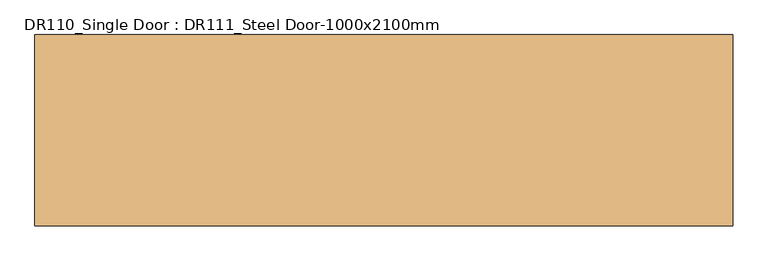
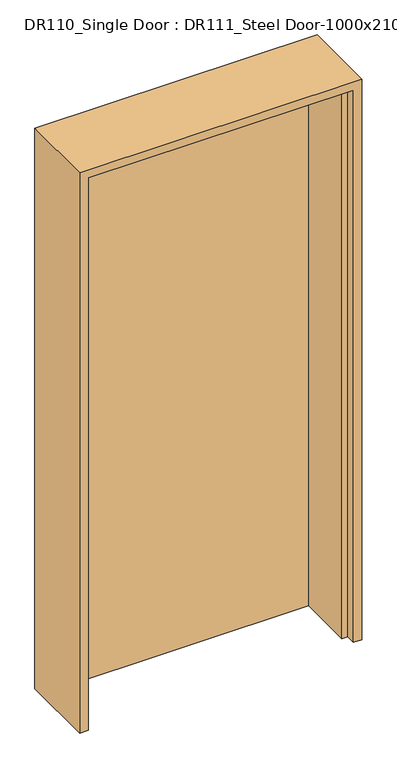
"""IFC4 building model written with IfcOpenShell, lengths in millimetres: door geometry, DR110_Single Door : DR111_Steel Door-1000x2100mm."""

import ifcopenshell
import ifcopenshell.guid

model = None  # the IFC model being written
_history = None  # IfcOwnerHistory: only IFC2X3 demands one
_inside = {}  # id of a spatial element -> (the spatial element, [elements in it])
_under = {}  # id of a project, library or spatial element -> (it, [spatial elements below it])
_declared = {}  # id of a project -> (the project, [libraries it declares])
_typed = {}  # id of a type object -> (the type object, [elements of that type])
_made_of = {}  # id of a material, layer set ... -> (it, [elements and type objects made of it])


def new_model(schema):
    """Start an empty IFC model of exactly this schema.

    Asked for "IFC4X3", IfcOpenShell would pick the latest addendum, in which some entities
    have other attributes; the version numbers below select the first issue.
    IFC2X3 requires an IfcOwnerHistory on every rooted entity: one is made here for all.
    """
    global model, _history
    if schema == "IFC4X3":
        model = ifcopenshell.file(schema_version=(4, 3, 0, 0))
    else:
        model = ifcopenshell.file(schema=schema)
    _inside.clear()
    _under.clear()
    _declared.clear()
    _typed.clear()
    _made_of.clear()
    _history = None
    if model.schema == "IFC2X3":
        org = make("IfcOrganization", Name="unknown")
        user = make(
            "IfcPersonAndOrganization",
            ThePerson=make("IfcPerson", FamilyName="unknown"),
            TheOrganization=org,
        )
        app = make(
            "IfcApplication",
            ApplicationDeveloper=org,
            Version="unknown",
            ApplicationFullName="unknown",
            ApplicationIdentifier="unknown",
        )
        _history = make(
            "IfcOwnerHistory",
            OwningUser=user,
            OwningApplication=app,
            ChangeAction="ADDED",
            CreationDate=0,
        )
    return model


def make(cls, **values):
    """One entity of the class cls with the attributes given. An attribute that is None is left unset."""
    return model.create_entity(
        cls, **{name: value for name, value in values.items() if value is not None}
    )


def rooted(cls, **values):
    """An entity with a GlobalId (a new one), such as an element, a storey or a relation."""
    return make(cls, GlobalId=ifcopenshell.guid.new(), OwnerHistory=_history, **values)


def si_unit(unit_type, name, prefix=None):
    """IfcSIUnit, for example si_unit("LENGTHUNIT", "METRE", prefix="MILLI")."""
    return make("IfcSIUnit", UnitType=unit_type, Prefix=prefix, Name=name)


def assignment(units):
    """IfcUnitAssignment: the units of a project."""
    return None if units is None else make("IfcUnitAssignment", Units=units)


def point(xyz):
    """IfcCartesianPoint."""
    return None if xyz is None else make("IfcCartesianPoint", Coordinates=xyz)


def direction(xyz):
    """IfcDirection."""
    return None if xyz is None else make("IfcDirection", DirectionRatios=xyz)


def frame(location, z_axis=None, x_axis=None):
    """IfcAxis2Placement3D, a coordinate frame: its origin and axes. An axis left out is left unset."""
    return make(
        "IfcAxis2Placement3D",
        Location=point(location),
        Axis=direction(z_axis),
        RefDirection=direction(x_axis),
    )


def origin():
    """The frame at (0, 0, 0) with its axes left unset."""
    return frame((0.0, 0.0, 0.0))


def origin_with_axes():
    """The frame at (0, 0, 0) with the z axis (0, 0, 1) and the x axis (1, 0, 0) written out."""
    return frame((0.0, 0.0, 0.0), z_axis=(0.0, 0.0, 1.0), x_axis=(1.0, 0.0, 0.0))


def place(relative_to, where):
    """IfcLocalPlacement: puts the frame where relative to a parent placement (None: the world)."""
    return make(
        "IfcLocalPlacement", PlacementRelTo=relative_to, RelativePlacement=where
    )


def context(
    kind, dimensions, precision=None, world=None, true_north=None, identifier=None
):
    """IfcGeometricRepresentationContext, for example the 3D "Model" context."""
    return make(
        "IfcGeometricRepresentationContext",
        ContextIdentifier=identifier,
        ContextType=kind,
        CoordinateSpaceDimension=dimensions,
        Precision=precision,
        WorldCoordinateSystem=world,
        TrueNorth=true_north,
    )


def project(units=None, contexts=None):
    """IfcProject with its units and contexts."""
    return rooted(
        "IfcProject",
        Name="project",
        RepresentationContexts=contexts,
        UnitsInContext=assignment(units),
    )


def spatial(cls, under=None, at=None, **own):
    """A site, building, storey or space (cls), placed at a placement, below another one or the project."""
    s = rooted(cls, ObjectPlacement=at, **own)
    if under is not None:
        _under.setdefault(under.id(), (under, []))[1].append(s)
    return s


def polyline(points):
    """IfcPolyline through the points."""
    return make("IfcPolyline", Points=[point(p) for p in points])


def outline(outer, holes=None, kind="AREA"):
    """IfcArbitraryClosedProfileDef: a profile drawn as a closed curve; with holes, ...WithVoids."""
    if holes is None:
        return make("IfcArbitraryClosedProfileDef", ProfileType=kind, OuterCurve=outer)
    return make(
        "IfcArbitraryProfileDefWithVoids",
        ProfileType=kind,
        OuterCurve=outer,
        InnerCurves=holes,
    )


def extrude(swept, where, along, depth):
    """IfcExtrudedAreaSolid: the profile swept, set in the frame where, extruded along a direction by depth."""
    return make(
        "IfcExtrudedAreaSolid",
        SweptArea=swept,
        Position=where,
        ExtrudedDirection=direction(along),
        Depth=depth,
    )


def faces_of(points, faces, orient=None, outer=None):
    """IfcFace entities. A face is a list of loops; a loop is a list of indices into points, from 0.

    orient and outer hold one flag for each loop. By default every Orientation is true, the
    first loop of a face is its IfcFaceOuterBound and the others are IfcFaceBound.
    """
    made = []
    for i, loops in enumerate(faces):
        bounds = []
        for j, loop in enumerate(loops):
            is_outer = j == 0 if outer is None else outer[i][j]
            bounds.append(
                make(
                    "IfcFaceOuterBound" if is_outer else "IfcFaceBound",
                    Bound=make("IfcPolyLoop", Polygon=[points[k] for k in loop]),
                    Orientation=True if orient is None else orient[i][j],
                )
            )
        made.append(make("IfcFace", Bounds=bounds))
    return made


def faceted_brep(points, faces, orient=None, outer=None, voids=None):
    """IfcFacetedBrep: a solid bounded by flat faces; with voids (closed shells), ...WithVoids."""
    shared = [point(p) for p in points]
    hull = make("IfcClosedShell", CfsFaces=faces_of(shared, faces, orient, outer))
    if voids is None:
        return make("IfcFacetedBrep", Outer=hull)
    return make(
        "IfcFacetedBrepWithVoids",
        Outer=hull,
        Voids=[
            make(cls, CfsFaces=faces_of(shared, fs, o, b)) for cls, fs, o, b in voids
        ],
    )


def shape(context_of_items, identifier, shape_type, items):
    """IfcShapeRepresentation: the items that make up one representation, for example the "Body"."""
    return make(
        "IfcShapeRepresentation",
        ContextOfItems=context_of_items,
        RepresentationIdentifier=identifier,
        RepresentationType=shape_type,
        Items=items,
    )


def source(mapping_origin, context_of_items, identifier, shape_type, items):
    """IfcRepresentationMap: a shape defined once, which mapped items show again and again."""
    return make(
        "IfcRepresentationMap",
        MappingOrigin=mapping_origin,
        MappedRepresentation=shape(context_of_items, identifier, shape_type, items),
    )


def transform(
    local_origin,
    x_axis=None,
    y_axis=None,
    z_axis=None,
    scale=None,
    scale2=None,
    scale3=None,
    uniform=True,
):
    """IfcCartesianTransformationOperator3D, or its non-uniform kind. x_axis, y_axis, z_axis: its Axis1, 2, 3."""
    if uniform:
        return make(
            "IfcCartesianTransformationOperator3D",
            Axis1=direction(x_axis),
            Axis2=direction(y_axis),
            LocalOrigin=point(local_origin),
            Scale=scale,
            Axis3=direction(z_axis),
        )
    return make(
        "IfcCartesianTransformationOperator3DnonUniform",
        Axis1=direction(x_axis),
        Axis2=direction(y_axis),
        LocalOrigin=point(local_origin),
        Scale=scale,
        Axis3=direction(z_axis),
        Scale2=scale2,
        Scale3=scale3,
    )


def mapped(mapping_source, mapping_target):
    """IfcMappedItem: shows the shape of a source again, moved by a transform."""
    return make(
        "IfcMappedItem", MappingSource=mapping_source, MappingTarget=mapping_target
    )


def made_of(thing, what):
    """Note that an element or type object is made of a material, layer set ...; save() writes the relation."""
    if what is not None:
        _made_of.setdefault(what.id(), (what, []))[1].append(thing)
    return thing


def element(
    cls,
    number,
    at=None,
    inside=None,
    cuts=None,
    type_object=None,
    material=None,
    context=None,
    identifier="Body",
    shape_type=None,
    held_by="IfcProductDefinitionShape",
    body=None,
    shapes=None,
    **own,
):
    """One element of the class cls, such as IfcWall. Its Tag is "e" and its number.

    at: its placement. inside: the storey or other place that contains it. cuts: it is an
    opening in that element (IfcRelVoidsElement). A single representation is given by context,
    identifier, shape_type and body (its items); several are given by shapes. held_by: the class
    of the entity that holds the representations. save() writes the other relations.
    """
    e = rooted(cls, Tag="e%d" % number, ObjectPlacement=at, **own)
    if body is not None:
        shapes = [shape(context, identifier, shape_type, body)]
    if shapes is not None:
        e.Representation = make(held_by, Representations=shapes)
    if inside is not None:
        _inside.setdefault(inside.id(), (inside, []))[1].append(e)
    if cuts is not None:
        rooted(
            "IfcRelVoidsElement", RelatingBuildingElement=cuts, RelatedOpeningElement=e
        )
    if type_object is not None:
        _typed.setdefault(type_object.id(), (type_object, []))[1].append(e)
    return made_of(e, material)


def aggregate(whole, parts):
    """IfcRelAggregates: a whole, such as a stair, and the parts it consists of."""
    return rooted("IfcRelAggregates", RelatingObject=whole, RelatedObjects=parts)


def save(model, path):
    """Write the relations noted so far, then the file.

    IfcRelAggregates (storeys below a building ...), IfcRelContainedInSpatialStructure (elements
    in a storey), IfcRelDefinesByType, IfcRelAssociatesMaterial and IfcRelDeclares: one each for
    every whole, place, type object, material and project.
    """
    for whole, parts in _under.values():
        aggregate(whole, parts)
    for where, things in _inside.values():
        rooted(
            "IfcRelContainedInSpatialStructure",
            RelatedElements=things,
            RelatingStructure=where,
        )
    for kind, things in _typed.values():
        rooted("IfcRelDefinesByType", RelatedObjects=things, RelatingType=kind)
    for what, things in _made_of.values():
        rooted("IfcRelAssociatesMaterial", RelatedObjects=things, RelatingMaterial=what)
    for by, libraries in _declared.values():
        rooted("IfcRelDeclares", RelatingContext=by, RelatedDefinitions=libraries)
    model.write(path)


def dr110_single_door_dr111_steel_door_1000x2100mm_d0b51d4b(model_context):
    return source(origin(), model_context, "Body", "SolidModel", [
        extrude(outline(polyline([(470.0, 137.0), (470.0, 102.0), (-470.0, 102.0), (-470.0, 137.0), (470.0, 137.0)])), origin_with_axes(), (0.0, 0.0, 1.0), 2070.0),
        faceted_brep([(470.0, 137.0, 0.0), (500.0, 137.0, 0.0), (500.0, -137.0, 0.0), (470.0, -137.0, 0.0), (470.0, -102.0, 0.0), (450.0, -102.0, 0.0), (450.0, 102.0, 0.0), (470.0, 102.0, 0.0), (470.0, 137.0, 2070.0), (-470.0, 137.0, 2070.0), (-470.0, 137.0, 0.0), (-500.0, 137.0, 0.0), (-500.0, 137.0, 2100.0), (500.0, 137.0, 2100.0), (500.0, -137.0, 2100.0), (-500.0, -137.0, 2100.0), (-500.0, -137.0, 0.0), (-470.0, -137.0, 0.0), (-470.0, -137.0, 2070.0), (470.0, -137.0, 2070.0), (470.0, -102.0, 2070.0), (-470.0, -102.0, 2070.0), (-470.0, -102.0, 0.0), (-450.0, -102.0, 0.0), (-450.0, -102.0, 2050.0), (450.0, -102.0, 2050.0), (450.0, 102.0, 2050.0), (-450.0, 102.0, 2050.0), (-450.0, 102.0, 0.0), (-470.0, 102.0, 0.0), (-470.0, 102.0, 2070.0), (470.0, 102.0, 2070.0)], [[[0, 1, 2, 3, 4, 5, 6, 7]], [[1, 0, 8, 9, 10, 11, 12, 13]], [[2, 1, 13, 14]], [[3, 2, 14, 15, 16, 17, 18, 19]], [[4, 3, 19, 20]], [[5, 4, 20, 21, 22, 23, 24, 25]], [[6, 5, 25, 26]], [[7, 6, 26, 27, 28, 29, 30, 31]], [[0, 7, 31, 8]], [[9, 30, 29, 10]], [[10, 29, 28, 23, 22, 17, 16, 11]], [[15, 12, 11, 16]], [[21, 18, 17, 22]], [[27, 24, 23, 28]], [[14, 13, 12, 15]], [[20, 19, 18, 21]], [[26, 25, 24, 27]], [[8, 31, 30, 9]]]),
    ])


if __name__ == "__main__":
    model = new_model("IFC4")
    model_context = context("Model", 3, world=origin())
    ifc_project = project(units=[si_unit("LENGTHUNIT", "METRE", prefix="MILLI")], contexts=[model_context])
    site = spatial("IfcSite", under=ifc_project)
    building = spatial("IfcBuilding", under=site)
    placement = place(None, origin())
    dr110_single_door_dr111_steel_door_1000x2100mm_shape = dr110_single_door_dr111_steel_door_1000x2100mm_d0b51d4b(model_context)
    element("IfcDoor", 1, ObjectType="DR110_Single Door : DR111_Steel Door-1000x2100mm", at=placement, inside=building, context=model_context, shape_type="MappedRepresentation", body=[
        mapped(dr110_single_door_dr111_steel_door_1000x2100mm_shape, transform((0.0, 0.0, 0.0), x_axis=(1.0, 0.0, 0.0), y_axis=(0.0, 1.0, 0.0), z_axis=(0.0, 0.0, 1.0))),
    ])
    save(model, "model.ifc")

# Revit data of these elements
# Type "DR110_Single Door : DR111_Steel Door-1000x2100mm"
#   Type Mark = "SD"
#   Analytic Construction = "<None>"
#   프레임 투영 외부. = 25 mm
#   프레임 투영 내부. = 25 mm
#   프레임 폭 = 75 mm
#   Height = 2100 mm
#   Width = 1000 mm
#   Define Thermal Properties by = 1
#   문 패널 = SD1 문 패널
#   문 프레임 = A04AQ098-00002_Steel Door_non FP_single
#   Function = (empty or 0)
#   Wall Closure = (empty or 0)
# Element 1 (IfcDoor, "DR110_Single Door : DR111_Steel Door-1000x2100mm")
#   Materials on its faces: "A04AQ098-00002_Steel Door_non FP_single", "SD1 문 패널"
# Materials
#   "SD1 문 패널": class "금속", colour RGB 247 247 247, transparency 0, Description = "STEEL DOOR (1000Wx2100H)"
#   "A04AQ098-00002_Steel Door_non FP_single": class "금속", colour RGB 247 247 247, transparency 0, Description = "Steel Door", W00) Work Master Code = "A04AQ098-00002", W01) Work Master_Lv1 = "Finishing Work", W02) Work Master_Lv2 = "Door & Window Work", W03) Work Master_Spec.1 = "Steel Door w/ Steel Frame", W04) Work Master_Spec.2 = "Fire Protective Rating: N/A, Single Door", W05) Work Master_Spec.3 = "w/ Hardware & Accessories", Cost = 0
